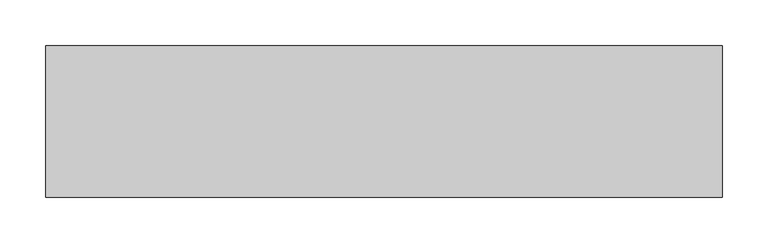
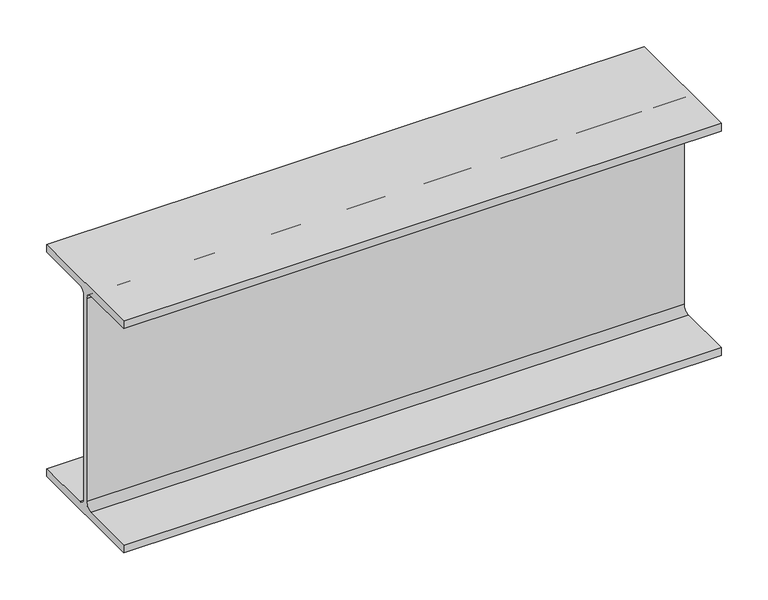
"""IFC4 building model written with IfcOpenShell, lengths in millimetres: beam geometry, Old_Steel Beam_H-KSD3502 : H_SB_ASB_H-300×300x10x15."""

from ifc_helpers import new_model, si_unit, point, frame, frame_2d, origin, place, context, project, spatial, polyline, circle_curve, trimmed, segment, composite_curve, outline, extrude, source, transform, mapped, element, save


def beam_189123d8(model_context):
    return source(origin(), model_context, "Body", "SweptSolid", [
        extrude(outline(composite_curve([segment(polyline([(82.5, -141.5), (82.5, -151.7), (-82.5, -151.7), (-82.5, -141.5), (-11.9, -141.5)]), True, "CONTINUOUS"), segment(trimmed(circle_curve(frame_2d((-11.9, -132.6)), 8.9), [point((-11.9, -141.5))], [point((-3.0, -132.6))], True, "CARTESIAN"), True, "CONTINUOUS"), segment(polyline([(-3.0, -132.6), (-3.0, 132.6)]), True, "CONTINUOUS"), segment(trimmed(circle_curve(frame_2d((-11.9, 132.6)), 8.9), [point((-3.0, 132.6))], [point((-11.9, 141.5))], True, "CARTESIAN"), True, "CONTINUOUS"), segment(polyline([(-11.9, 141.5), (-82.5, 141.5), (-82.5, 151.7), (82.5, 151.7), (82.5, 141.5), (11.9, 141.5)]), True, "CONTINUOUS"), segment(trimmed(circle_curve(frame_2d((11.9, 132.6)), 8.9), [point((11.9, 141.5))], [point((3.0, 132.6))], True, "CARTESIAN"), True, "CONTINUOUS"), segment(polyline([(3.0, 132.6), (3.0, -132.6)]), True, "CONTINUOUS"), segment(trimmed(circle_curve(frame_2d((11.9, -132.6)), 8.9), [point((3.0, -132.6))], [point((11.9, -141.5))], True, "CARTESIAN"), True, "CONTINUOUS"), segment(polyline([(11.9, -141.5), (82.5, -141.5)]), True, "CONTINUOUS")], self_intersect=False)), frame((-502.4937811, 0.0, 0.0), z_axis=(1.0, 0.0, 0.0), x_axis=(0.0, 1.0, 0.0)), (0.0, 0.0, 1.0), 738.1005223),
    ])


if __name__ == "__main__":
    model = new_model("IFC4")
    model_context = context("Model", 3, world=origin())
    ifc_project = project(units=[si_unit("LENGTHUNIT", "METRE", prefix="MILLI")], contexts=[model_context])
    site = spatial("IfcSite", under=ifc_project)
    building = spatial("IfcBuilding", under=site)
    placement = place(None, origin())
    beam_shape = beam_189123d8(model_context)
    element("IfcBeam", 1, ObjectType="Old_Steel Beam_H-KSD3502 : H_SB_ASB_H-300×300x10x15", at=placement, inside=building, context=model_context, shape_type="MappedRepresentation", body=[
        mapped(beam_shape, transform((0.0, 0.0, 0.0), x_axis=(1.0, 0.0, 0.0), y_axis=(0.0, 1.0, 0.0), z_axis=(0.0, 0.0, 1.0))),
    ])
    save(model, "model.ifc")

# Revit data of these elements
# Type "Old_Steel Beam_H-KSD3502 : H_SB_ASB_H-300×300x10x15"
#   Width = 30.0 cm
#   Web Thickness = 1.0 cm
#   Web Fillet = 1.8 cm
#   Warping Constant = 1370670.0 cm⁶
#   Torsional Moment of Inertia = 77.00 cm⁴
#   Torsional Modulus = 1.0 cm³
#   Section Area = 119.8 cm²
#   Plastic Modulus weak axis = 684.0 cm³
#   Plastic Modulus strong axis = 1500.0 cm³
#   Perimeter = 1.75 m²/m
#   Nominal Weight = 94.00 kgf/m
#   Moment of Inertia weak axis = 6750.00 cm⁴
#   Moment of Inertia strong axis = 20400.00 cm⁴
#   Height = 30.0 cm
#   Flange Thickness = 1.5 cm
#   Elastic Modulus weak axis = 450.0 cm³
#   Elastic Modulus strong axis = 1360.0 cm³
#   Centroid Vertical = 15.0 cm
#   Centroid Horizontal = 15.0 cm
#   Length [instance default] = 1.5240 m
#   Structural Material [instance default] = Steel, 45-345
#   Assembly Code = ""
# Element 1 (IfcBeam, "Old_Steel Beam_H-KSD3502 : H_SB_ASB_H-300×300x10x15")
#   Structural Material = none
# Materials
#   "Steel, 45-345": class "Metal", colour RGB 189 187 185, transparency 0, Description = "Steel 345 MPa", Cost = 0
